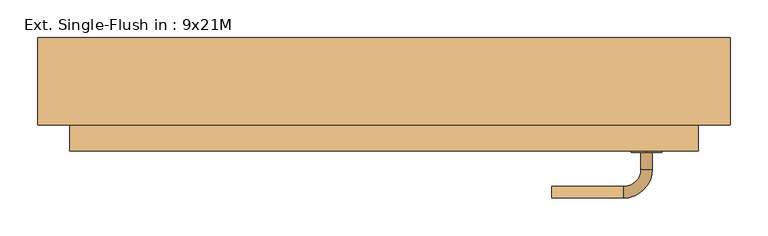
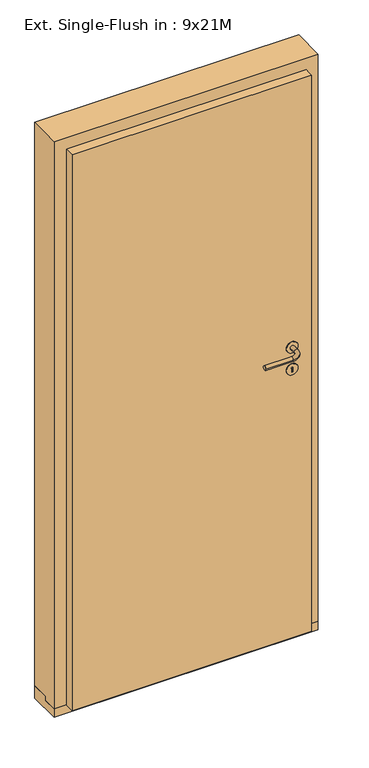
"""IFC4 building model written with IfcOpenShell, lengths in millimetres: door geometry, Ext. Single-Flush in : 9x21M."""

import ifcopenshell
import ifcopenshell.guid

model = None  # the IFC model being written
_history = None  # IfcOwnerHistory: only IFC2X3 demands one
_inside = {}  # id of a spatial element -> (the spatial element, [elements in it])
_under = {}  # id of a project, library or spatial element -> (it, [spatial elements below it])
_declared = {}  # id of a project -> (the project, [libraries it declares])
_typed = {}  # id of a type object -> (the type object, [elements of that type])
_made_of = {}  # id of a material, layer set ... -> (it, [elements and type objects made of it])


def new_model(schema):
    """Start an empty IFC model of exactly this schema.

    Asked for "IFC4X3", IfcOpenShell would pick the latest addendum, in which some entities
    have other attributes; the version numbers below select the first issue.
    IFC2X3 requires an IfcOwnerHistory on every rooted entity: one is made here for all.
    """
    global model, _history
    if schema == "IFC4X3":
        model = ifcopenshell.file(schema_version=(4, 3, 0, 0))
    else:
        model = ifcopenshell.file(schema=schema)
    _inside.clear()
    _under.clear()
    _declared.clear()
    _typed.clear()
    _made_of.clear()
    _history = None
    if model.schema == "IFC2X3":
        org = make("IfcOrganization", Name="unknown")
        user = make(
            "IfcPersonAndOrganization",
            ThePerson=make("IfcPerson", FamilyName="unknown"),
            TheOrganization=org,
        )
        app = make(
            "IfcApplication",
            ApplicationDeveloper=org,
            Version="unknown",
            ApplicationFullName="unknown",
            ApplicationIdentifier="unknown",
        )
        _history = make(
            "IfcOwnerHistory",
            OwningUser=user,
            OwningApplication=app,
            ChangeAction="ADDED",
            CreationDate=0,
        )
    return model


def make(cls, **values):
    """One entity of the class cls with the attributes given. An attribute that is None is left unset."""
    return model.create_entity(
        cls, **{name: value for name, value in values.items() if value is not None}
    )


def rooted(cls, **values):
    """An entity with a GlobalId (a new one), such as an element, a storey or a relation."""
    return make(cls, GlobalId=ifcopenshell.guid.new(), OwnerHistory=_history, **values)


def si_unit(unit_type, name, prefix=None):
    """IfcSIUnit, for example si_unit("LENGTHUNIT", "METRE", prefix="MILLI")."""
    return make("IfcSIUnit", UnitType=unit_type, Prefix=prefix, Name=name)


def assignment(units):
    """IfcUnitAssignment: the units of a project."""
    return None if units is None else make("IfcUnitAssignment", Units=units)


def point(xyz):
    """IfcCartesianPoint."""
    return None if xyz is None else make("IfcCartesianPoint", Coordinates=xyz)


def direction(xyz):
    """IfcDirection."""
    return None if xyz is None else make("IfcDirection", DirectionRatios=xyz)


def frame(location, z_axis=None, x_axis=None):
    """IfcAxis2Placement3D, a coordinate frame: its origin and axes. An axis left out is left unset."""
    return make(
        "IfcAxis2Placement3D",
        Location=point(location),
        Axis=direction(z_axis),
        RefDirection=direction(x_axis),
    )


def frame_2d(location, x_axis=None):
    """IfcAxis2Placement2D, a coordinate frame in the plane: its origin and x axis."""
    return make(
        "IfcAxis2Placement2D", Location=point(location), RefDirection=direction(x_axis)
    )


def origin():
    """The frame at (0, 0, 0) with its axes left unset."""
    return frame((0.0, 0.0, 0.0))


def place(relative_to, where):
    """IfcLocalPlacement: puts the frame where relative to a parent placement (None: the world)."""
    return make(
        "IfcLocalPlacement", PlacementRelTo=relative_to, RelativePlacement=where
    )


def context(
    kind, dimensions, precision=None, world=None, true_north=None, identifier=None
):
    """IfcGeometricRepresentationContext, for example the 3D "Model" context."""
    return make(
        "IfcGeometricRepresentationContext",
        ContextIdentifier=identifier,
        ContextType=kind,
        CoordinateSpaceDimension=dimensions,
        Precision=precision,
        WorldCoordinateSystem=world,
        TrueNorth=true_north,
    )


def project(units=None, contexts=None):
    """IfcProject with its units and contexts."""
    return rooted(
        "IfcProject",
        Name="project",
        RepresentationContexts=contexts,
        UnitsInContext=assignment(units),
    )


def spatial(cls, under=None, at=None, **own):
    """A site, building, storey or space (cls), placed at a placement, below another one or the project."""
    s = rooted(cls, ObjectPlacement=at, **own)
    if under is not None:
        _under.setdefault(under.id(), (under, []))[1].append(s)
    return s


def polyline(points):
    """IfcPolyline through the points."""
    return make("IfcPolyline", Points=[point(p) for p in points])


def circle_curve(where, radius):
    """IfcCircle in the frame where."""
    return make("IfcCircle", Position=where, Radius=radius)


def ellipse_curve(where, semi_axis1, semi_axis2):
    """IfcEllipse in the frame where."""
    return make(
        "IfcEllipse", Position=where, SemiAxis1=semi_axis1, SemiAxis2=semi_axis2
    )


def trimmed(basis, trim1, trim2, sense, master):
    """IfcTrimmedCurve: the piece of a basis curve between two trims."""
    return make(
        "IfcTrimmedCurve",
        BasisCurve=basis,
        Trim1=trim1,
        Trim2=trim2,
        SenseAgreement=sense,
        MasterRepresentation=master,
    )


def segment(curve, same_sense, transition):
    """IfcCompositeCurveSegment."""
    return make(
        "IfcCompositeCurveSegment",
        Transition=transition,
        SameSense=same_sense,
        ParentCurve=curve,
    )


def composite_curve(segments, self_intersect=None):
    """IfcCompositeCurve: segments joined end to end."""
    return make("IfcCompositeCurve", Segments=segments, SelfIntersect=self_intersect)


def outline(outer, holes=None, kind="AREA"):
    """IfcArbitraryClosedProfileDef: a profile drawn as a closed curve; with holes, ...WithVoids."""
    if holes is None:
        return make("IfcArbitraryClosedProfileDef", ProfileType=kind, OuterCurve=outer)
    return make(
        "IfcArbitraryProfileDefWithVoids",
        ProfileType=kind,
        OuterCurve=outer,
        InnerCurves=holes,
    )


def extrude(swept, where, along, depth):
    """IfcExtrudedAreaSolid: the profile swept, set in the frame where, extruded along a direction by depth."""
    return make(
        "IfcExtrudedAreaSolid",
        SweptArea=swept,
        Position=where,
        ExtrudedDirection=direction(along),
        Depth=depth,
    )


def faces_of(points, faces, orient=None, outer=None):
    """IfcFace entities. A face is a list of loops; a loop is a list of indices into points, from 0.

    orient and outer hold one flag for each loop. By default every Orientation is true, the
    first loop of a face is its IfcFaceOuterBound and the others are IfcFaceBound.
    """
    made = []
    for i, loops in enumerate(faces):
        bounds = []
        for j, loop in enumerate(loops):
            is_outer = j == 0 if outer is None else outer[i][j]
            bounds.append(
                make(
                    "IfcFaceOuterBound" if is_outer else "IfcFaceBound",
                    Bound=make("IfcPolyLoop", Polygon=[points[k] for k in loop]),
                    Orientation=True if orient is None else orient[i][j],
                )
            )
        made.append(make("IfcFace", Bounds=bounds))
    return made


def faceted_brep(points, faces, orient=None, outer=None, voids=None):
    """IfcFacetedBrep: a solid bounded by flat faces; with voids (closed shells), ...WithVoids."""
    shared = [point(p) for p in points]
    hull = make("IfcClosedShell", CfsFaces=faces_of(shared, faces, orient, outer))
    if voids is None:
        return make("IfcFacetedBrep", Outer=hull)
    return make(
        "IfcFacetedBrepWithVoids",
        Outer=hull,
        Voids=[
            make(cls, CfsFaces=faces_of(shared, fs, o, b)) for cls, fs, o, b in voids
        ],
    )


def shape(context_of_items, identifier, shape_type, items):
    """IfcShapeRepresentation: the items that make up one representation, for example the "Body"."""
    return make(
        "IfcShapeRepresentation",
        ContextOfItems=context_of_items,
        RepresentationIdentifier=identifier,
        RepresentationType=shape_type,
        Items=items,
    )


def source(mapping_origin, context_of_items, identifier, shape_type, items):
    """IfcRepresentationMap: a shape defined once, which mapped items show again and again."""
    return make(
        "IfcRepresentationMap",
        MappingOrigin=mapping_origin,
        MappedRepresentation=shape(context_of_items, identifier, shape_type, items),
    )


def transform(
    local_origin,
    x_axis=None,
    y_axis=None,
    z_axis=None,
    scale=None,
    scale2=None,
    scale3=None,
    uniform=True,
):
    """IfcCartesianTransformationOperator3D, or its non-uniform kind. x_axis, y_axis, z_axis: its Axis1, 2, 3."""
    if uniform:
        return make(
            "IfcCartesianTransformationOperator3D",
            Axis1=direction(x_axis),
            Axis2=direction(y_axis),
            LocalOrigin=point(local_origin),
            Scale=scale,
            Axis3=direction(z_axis),
        )
    return make(
        "IfcCartesianTransformationOperator3DnonUniform",
        Axis1=direction(x_axis),
        Axis2=direction(y_axis),
        LocalOrigin=point(local_origin),
        Scale=scale,
        Axis3=direction(z_axis),
        Scale2=scale2,
        Scale3=scale3,
    )


def mapped(mapping_source, mapping_target):
    """IfcMappedItem: shows the shape of a source again, moved by a transform."""
    return make(
        "IfcMappedItem", MappingSource=mapping_source, MappingTarget=mapping_target
    )


def made_of(thing, what):
    """Note that an element or type object is made of a material, layer set ...; save() writes the relation."""
    if what is not None:
        _made_of.setdefault(what.id(), (what, []))[1].append(thing)
    return thing


def element(
    cls,
    number,
    at=None,
    inside=None,
    cuts=None,
    type_object=None,
    material=None,
    context=None,
    identifier="Body",
    shape_type=None,
    held_by="IfcProductDefinitionShape",
    body=None,
    shapes=None,
    **own,
):
    """One element of the class cls, such as IfcWall. Its Tag is "e" and its number.

    at: its placement. inside: the storey or other place that contains it. cuts: it is an
    opening in that element (IfcRelVoidsElement). A single representation is given by context,
    identifier, shape_type and body (its items); several are given by shapes. held_by: the class
    of the entity that holds the representations. save() writes the other relations.
    """
    e = rooted(cls, Tag="e%d" % number, ObjectPlacement=at, **own)
    if body is not None:
        shapes = [shape(context, identifier, shape_type, body)]
    if shapes is not None:
        e.Representation = make(held_by, Representations=shapes)
    if inside is not None:
        _inside.setdefault(inside.id(), (inside, []))[1].append(e)
    if cuts is not None:
        rooted(
            "IfcRelVoidsElement", RelatingBuildingElement=cuts, RelatedOpeningElement=e
        )
    if type_object is not None:
        _typed.setdefault(type_object.id(), (type_object, []))[1].append(e)
    return made_of(e, material)


def aggregate(whole, parts):
    """IfcRelAggregates: a whole, such as a stair, and the parts it consists of."""
    return rooted("IfcRelAggregates", RelatingObject=whole, RelatedObjects=parts)


def save(model, path):
    """Write the relations noted so far, then the file.

    IfcRelAggregates (storeys below a building ...), IfcRelContainedInSpatialStructure (elements
    in a storey), IfcRelDefinesByType, IfcRelAssociatesMaterial and IfcRelDeclares: one each for
    every whole, place, type object, material and project.
    """
    for whole, parts in _under.values():
        aggregate(whole, parts)
    for where, things in _inside.values():
        rooted(
            "IfcRelContainedInSpatialStructure",
            RelatedElements=things,
            RelatingStructure=where,
        )
    for kind, things in _typed.values():
        rooted("IfcRelDefinesByType", RelatedObjects=things, RelatingType=kind)
    for what, things in _made_of.values():
        rooted("IfcRelAssociatesMaterial", RelatedObjects=things, RelatingMaterial=what)
    for by, libraries in _declared.values():
        rooted("IfcRelDeclares", RelatingContext=by, RelatedDefinitions=libraries)
    model.write(path)


def plane_surface(at):
    """IfcPlane: the flat surface through the origin of the frame at, square to its z axis."""
    return make("IfcPlane", Position=at)


def cylinder_surface(at, radius):
    """IfcCylindricalSurface: all points at the distance radius from the z axis of the frame at."""
    return make("IfcCylindricalSurface", Position=at, Radius=radius)


def revolved_surface(curve, axis_point, axis_direction):
    """IfcSurfaceOfRevolution: the curve turned about the line through axis_point along axis_direction."""
    return make(
        "IfcSurfaceOfRevolution",
        SweptCurve=make("IfcArbitraryOpenProfileDef", ProfileType="CURVE", Curve=curve),
        AxisPosition=make("IfcAxis1Placement", Location=point(axis_point), Axis=direction(axis_direction)),
    )


def advanced_brep(points, edges, surfaces, faces):
    """IfcAdvancedBrep: a solid bounded by faces that lie on surfaces and meet in shared edges.

    An edge is (start, end): straight between two places in points (the first is 0);
    or (start, end, curve); or (start, end, curve, False) where it runs against its curve.
    A face is (place in surfaces, loops), or (place, loops, False) where it looks against
    its surface's normal. A loop lists edges by number (the first is 1), with a minus sign
    where the edge is run from its end to its start. The first loop is the outer one.
    """
    corners = [point(p) for p in points]
    vertices = [make("IfcVertexPoint", VertexGeometry=c) for c in corners]
    made = []
    for start, end, *more in edges:
        made.append(
            make(
                "IfcEdgeCurve",
                EdgeStart=vertices[start],
                EdgeEnd=vertices[end],
                EdgeGeometry=more[0] if more else make("IfcPolyline", Points=[corners[start], corners[end]]),
                SameSense=more[1] if len(more) > 1 else True,
            )
        )
    hull = []
    for where, loops, *sense in faces:
        bounds = []
        for j, loop in enumerate(loops):
            ring = [make("IfcOrientedEdge", EdgeElement=made[abs(k) - 1], Orientation=k > 0) for k in loop]
            bounds.append(
                make(
                    "IfcFaceOuterBound" if j == 0 else "IfcFaceBound",
                    Bound=make("IfcEdgeLoop", EdgeList=ring),
                    Orientation=True,
                )
            )
        hull.append(make("IfcAdvancedFace", Bounds=bounds, FaceSurface=surfaces[where], SameSense=sense[0] if sense else True))
    return make("IfcAdvancedBrep", Outer=make("IfcClosedShell", CfsFaces=hull))


def ext_single_flush_in_9x21m_d6ab10a1(model_context):
    return source(origin(), model_context, "Body", "SolidModel", [
        extrude(outline(composite_curve([segment(trimmed(circle_curve(frame_2d((1090.0, 346.0)), 20.0), [point((1070.0, 346.0))], [point((1110.0, 346.0))], False, "CARTESIAN"), True, "CONTINUOUS"), segment(trimmed(circle_curve(frame_2d((1090.0, 346.0)), 20.0), [point((1110.0, 346.0))], [point((1070.0, 346.0))], False, "CARTESIAN"), True, "CONTINUOUS")], self_intersect=False)), frame((0.0, 33.0, 0.0), z_axis=(0.0, 1.0, 0.0), x_axis=(0.0, 0.0, 1.0)), (0.0, 0.0, 1.0), 2.0),
        advanced_brep(
        [(353.5, 33.0, 1090.0), (338.5, 33.0, 1090.0), (353.5, 10.5, 1090.0), (338.5, 10.5, 1090.0), (316.0, -12.0, 1090.0), (316.0, -27.0, 1090.0), (221.0, -27.0, 1090.0), (221.0, -12.0, 1090.0)],
        [
            (0, 1, circle_curve(frame((346.0, 33.0, 1090.0), z_axis=(0.0, 1.0, 0.0), x_axis=(-1.0, 0.0, 0.0)), 7.5)),
            (1, 0, circle_curve(frame((346.0, 33.0, 1090.0), z_axis=(0.0, 1.0, 0.0), x_axis=(-1.0, 0.0, 0.0)), 7.5)),
            (0, 2),
            (2, 3, circle_curve(frame((346.0, 10.5, 1090.0), z_axis=(0.0, 1.0, 0.0), x_axis=(-1.0, 0.0, 0.0)), 7.5)),
            (3, 1),
            (3, 2, circle_curve(frame((346.0, 10.5, 1090.0), z_axis=(0.0, 1.0, 0.0), x_axis=(-1.0, 0.0, 0.0)), 7.5)),
            (4, 3, circle_curve(frame((316.0, 10.5, 1090.0), z_axis=(0.0, 0.0, 1.0), x_axis=(1.0, 0.0, 0.0)), 22.5)),
            (2, 5, circle_curve(frame((316.0, 10.5, 1090.0), z_axis=(0.0, 0.0, -1.0), x_axis=(1.0, 0.0, 0.0)), 37.5)),
            (5, 4, circle_curve(frame((316.0, -19.5, 1090.0), z_axis=(1.0, 0.0, 0.0), x_axis=(0.0, 1.0, 0.0)), 7.5)),
            (4, 5, circle_curve(frame((316.0, -19.5, 1090.0), z_axis=(1.0, 0.0, 0.0), x_axis=(0.0, 1.0, 0.0)), 7.5)),
            (5, 6),
            (6, 7, circle_curve(frame((221.0, -19.5, 1090.0), z_axis=(1.0, 0.0, 0.0), x_axis=(0.0, 1.0, 0.0)), 7.5)),
            (7, 4),
            (7, 6, circle_curve(frame((221.0, -19.5, 1090.0), z_axis=(1.0, 0.0, 0.0), x_axis=(0.0, 1.0, 0.0)), 7.5)),
        ],
        [
            plane_surface(frame((346.0, 33.0, 1090.0), z_axis=(0.0, 1.0, 0.0), x_axis=(0.0, 0.0, -1.0))),
            cylinder_surface(frame((346.0, 33.0, 1090.0), z_axis=(0.0, 1.0, 0.0), x_axis=(-1.0, 0.0, 0.0)), 7.5),
            revolved_surface(trimmed(ellipse_curve(frame((346.0, 10.5, 1090.0), z_axis=(0.0, 1.0, 0.0), x_axis=(-1.0, 0.0, 0.0)), 7.5, 7.5), [point((353.5, 10.5, 1090.0))], [point((338.5, 10.5, 1090.0))], True, "CARTESIAN"), (316.0, 10.5, 1090.0), (0.0, 0.0, -1.0)),
            revolved_surface(trimmed(ellipse_curve(frame((346.0, 10.5, 1090.0), z_axis=(0.0, 1.0, 0.0), x_axis=(-1.0, 0.0, 0.0)), 7.5, 7.5), [point((338.5, 10.5, 1090.0))], [point((353.5, 10.5, 1090.0))], True, "CARTESIAN"), (316.0, 10.5, 1090.0), (0.0, 0.0, -1.0)),
            cylinder_surface(frame((316.0, -19.5, 1090.0), z_axis=(1.0, 0.0, 0.0), x_axis=(0.0, 1.0, 0.0)), 7.5),
            plane_surface(frame((221.0, -19.5, 1090.0), z_axis=(-1.0, 0.0, 0.0), x_axis=(0.0, 0.0, -1.0))),
        ],
        [
            (0, [[1, 2]]),
            (1, [[-1, 3, 4, 5]]),
            (1, [[-2, -5, 6, -3]]),
            (2, [[7, -4, 8, 9]]),
            (3, [[-8, -6, -7, 10]]),
            (4, [[-9, 11, 12, 13]]),
            (4, [[-10, -13, 14, -11]]),
            (5, [[-14, -12]]),
        ],
    ),
        extrude(outline(composite_curve([segment(trimmed(circle_curve(frame_2d((1010.0, 346.0)), 20.0), [point((990.0, 346.0))], [point((1030.0, 346.0))], False, "CARTESIAN"), True, "CONTINUOUS"), segment(trimmed(circle_curve(frame_2d((1010.0, 346.0)), 20.0), [point((1030.0, 346.0))], [point((990.0, 346.0))], False, "CARTESIAN"), True, "CONTINUOUS")], self_intersect=False), holes=[composite_curve([segment(polyline([(1012.4019238, 347.5), (1000.0, 347.5), (1000.0, 344.5), (1012.4019238, 344.5)]), True, "CONTINUOUS"), segment(trimmed(circle_curve(frame_2d((1015.0, 346.0)), 3.0), [point((1012.4019238, 344.5))], [point((1012.4019238, 347.5))], True, "CARTESIAN"), True, "CONTINUOUS")], self_intersect=False)]), frame((0.0, 33.0, 0.0), z_axis=(0.0, 1.0, 0.0), x_axis=(0.0, 0.0, 1.0)), (0.0, 0.0, 1.0), 2.0),
        extrude(outline(composite_curve([segment(trimmed(circle_curve(frame_2d((1090.0, 346.0)), 20.0), [point((1070.0, 346.0))], [point((1110.0, 346.0))], False, "CARTESIAN"), True, "CONTINUOUS"), segment(trimmed(circle_curve(frame_2d((1090.0, 346.0)), 20.0), [point((1110.0, 346.0))], [point((1070.0, 346.0))], False, "CARTESIAN"), True, "CONTINUOUS")], self_intersect=False)), frame((0.0, 85.0, 0.0), z_axis=(0.0, 1.0, 0.0), x_axis=(0.0, 0.0, 1.0)), (0.0, 0.0, 1.0), 2.0),
        advanced_brep(
        [(353.5, 87.0, 1090.0), (338.5, 87.0, 1090.0), (338.5, 109.5, 1090.0), (353.5, 109.5, 1090.0), (316.0, 132.0, 1090.0), (316.0, 147.0, 1090.0), (221.0, 132.0, 1090.0), (221.0, 147.0, 1090.0)],
        [
            (0, 1, circle_curve(frame((346.0, 87.0, 1090.0), z_axis=(0.0, -1.0, 0.0), x_axis=(-1.0, 0.0, 0.0)), 7.5)),
            (1, 0, circle_curve(frame((346.0, 87.0, 1090.0), z_axis=(0.0, -1.0, 0.0), x_axis=(-1.0, 0.0, 0.0)), 7.5)),
            (1, 2),
            (2, 3, circle_curve(frame((346.0, 109.5, 1090.0), z_axis=(0.0, -1.0, 0.0), x_axis=(-1.0, 0.0, 0.0)), 7.5)),
            (3, 0),
            (3, 2, circle_curve(frame((346.0, 109.5, 1090.0), z_axis=(0.0, -1.0, 0.0), x_axis=(-1.0, 0.0, 0.0)), 7.5)),
            (4, 5, circle_curve(frame((316.0, 139.5, 1090.0), z_axis=(1.0, 0.0, 0.0), x_axis=(0.0, -1.0, 0.0)), 7.5)),
            (5, 3, circle_curve(frame((316.0, 109.5, 1090.0), z_axis=(0.0, 0.0, -1.0), x_axis=(1.0, 0.0, 0.0)), 37.5)),
            (2, 4, circle_curve(frame((316.0, 109.5, 1090.0), z_axis=(0.0, 0.0, 1.0), x_axis=(1.0, 0.0, 0.0)), 22.5)),
            (5, 4, circle_curve(frame((316.0, 139.5, 1090.0), z_axis=(1.0, 0.0, 0.0), x_axis=(0.0, -1.0, 0.0)), 7.5)),
            (4, 6),
            (6, 7, circle_curve(frame((221.0, 139.5, 1090.0), z_axis=(1.0, 0.0, 0.0), x_axis=(0.0, -1.0, 0.0)), 7.5)),
            (7, 5),
            (7, 6, circle_curve(frame((221.0, 139.5, 1090.0), z_axis=(1.0, 0.0, 0.0), x_axis=(0.0, -1.0, 0.0)), 7.5)),
        ],
        [
            plane_surface(frame((346.0, 87.0, 1090.0), z_axis=(0.0, -1.0, 0.0), x_axis=(0.0, 0.0, -1.0))),
            cylinder_surface(frame((346.0, 87.0, 1090.0), z_axis=(0.0, -1.0, 0.0), x_axis=(-1.0, 0.0, 0.0)), 7.5),
            revolved_surface(trimmed(ellipse_curve(frame((346.0, 109.5, 1090.0), z_axis=(0.0, 1.0, 0.0), x_axis=(-1.0, 0.0, 0.0)), 7.5, 7.5), [point((353.5, 109.5, 1090.0))], [point((338.5, 109.5, 1090.0))], True, "CARTESIAN"), (316.0, 109.5, 1090.0), (0.0, 0.0, -1.0)),
            revolved_surface(trimmed(ellipse_curve(frame((346.0, 109.5, 1090.0), z_axis=(0.0, 1.0, 0.0), x_axis=(-1.0, 0.0, 0.0)), 7.5, 7.5), [point((338.5, 109.5, 1090.0))], [point((353.5, 109.5, 1090.0))], True, "CARTESIAN"), (316.0, 109.5, 1090.0), (0.0, 0.0, -1.0)),
            cylinder_surface(frame((316.0, 139.5, 1090.0), z_axis=(1.0, 0.0, 0.0), x_axis=(0.0, -1.0, 0.0)), 7.5),
            plane_surface(frame((221.0, 139.5, 1090.0), z_axis=(-1.0, 0.0, 0.0), x_axis=(0.0, 0.0, -1.0))),
        ],
        [
            (0, [[1, 2]]),
            (1, [[3, 4, 5, -2]]),
            (1, [[-5, 6, -3, -1]]),
            (2, [[7, 8, -4, 9]]),
            (3, [[10, -9, -6, -8]]),
            (4, [[11, 12, 13, -7]]),
            (4, [[-13, 14, -11, -10]]),
            (5, [[-12, -14]]),
        ],
    ),
        extrude(outline(composite_curve([segment(trimmed(circle_curve(frame_2d((1010.0, 346.0)), 20.0), [point((990.0, 346.0))], [point((1030.0, 346.0))], False, "CARTESIAN"), True, "CONTINUOUS"), segment(trimmed(circle_curve(frame_2d((1010.0, 346.0)), 20.0), [point((1030.0, 346.0))], [point((990.0, 346.0))], False, "CARTESIAN"), True, "CONTINUOUS")], self_intersect=False), holes=[composite_curve([segment(polyline([(1012.4019238, 347.5), (1000.0, 347.5), (1000.0, 344.5), (1012.4019238, 344.5)]), True, "CONTINUOUS"), segment(trimmed(circle_curve(frame_2d((1015.0, 346.0)), 3.0), [point((1012.4019238, 344.5))], [point((1012.4019238, 347.5))], True, "CARTESIAN"), True, "CONTINUOUS")], self_intersect=False)]), frame((0.0, 85.0, 0.0), z_axis=(0.0, 1.0, 0.0), x_axis=(0.0, 0.0, 1.0)), (0.0, 0.0, 1.0), 2.0),
        faceted_brep([(-414.0, 69.0, 2058.0), (414.0, 69.0, 2058.0), (414.0, 69.0, 30.0), (456.0, 69.0, 30.0), (456.0, 69.0, 2100.0), (-456.0, 69.0, 2100.0), (-456.0, 69.0, 30.0), (-414.0, 69.0, 30.0), (414.0, 119.0, 2058.0), (414.0, 119.0, 45.0), (414.0, 119.0, 30.0), (-456.0, 119.0, 30.0), (-414.0, 119.0, 30.0), (456.0, 119.0, 30.0), (456.0, 184.0, 2100.0), (456.0, 119.0, 45.0), (456.0, 184.0, 45.0), (-456.0, 184.0, 2100.0), (-456.0, 184.0, 45.0), (-456.0, 119.0, 45.0), (-414.0, 119.0, 2058.0), (-414.0, 119.0, 45.0), (399.0, 184.0, 45.0), (399.0, 184.0, 2043.0), (-399.0, 184.0, 2043.0), (-399.0, 184.0, 45.0), (-399.0, 119.0, 45.0), (399.0, 119.0, 45.0), (399.0, 119.0, 2043.0), (-399.0, 119.0, 2043.0)], [[[0, 1, 2, 3, 4, 5, 6, 7]], [[1, 8, 9, 10, 2]], [[11, 12, 7, 6]], [[10, 13, 3, 2]], [[14, 4, 3, 13, 15, 16]], [[5, 17, 18, 19, 11, 6]], [[20, 0, 7, 12, 21]], [[17, 14, 16, 22, 23, 24, 25, 18]], [[21, 19, 18, 25, 26]], [[15, 9, 27, 22, 16]], [[12, 11, 19, 21]], [[13, 10, 9, 15]], [[28, 23, 22, 27]], [[24, 29, 26, 25]], [[29, 28, 27, 9, 8, 20, 21, 26]], [[5, 4, 14, 17]], [[24, 23, 28, 29]], [[1, 0, 20, 8]]]),
        extrude(outline(polyline([(-414.0, 85.0), (414.0, 85.0), (414.0, 35.0), (-414.0, 35.0), (-414.0, 85.0)])), frame((0.0, 0.0, 30.0), z_axis=(0.0, 0.0, 1.0), x_axis=(1.0, 0.0, 0.0)), (0.0, 0.0, 1.0), 2028.0),
        extrude(outline(polyline([(69.0, 30.0), (119.0, 30.0), (119.0, 45.0), (184.0, 45.0), (184.0, 0.0), (69.0, 0.0), (69.0, 30.0)])), frame((-456.0, 0.0, 0.0), z_axis=(1.0, 0.0, 0.0), x_axis=(0.0, 1.0, 0.0)), (0.0, 0.0, 1.0), 912.0),
    ])


if __name__ == "__main__":
    model = new_model("IFC4")
    model_context = context("Model", 3, world=origin())
    ifc_project = project(units=[si_unit("LENGTHUNIT", "METRE", prefix="MILLI")], contexts=[model_context])
    site = spatial("IfcSite", under=ifc_project)
    building = spatial("IfcBuilding", under=site)
    placement = place(None, origin())
    ext_single_flush_in_9x21m_shape = ext_single_flush_in_9x21m_d6ab10a1(model_context)
    element("IfcDoor", 1, ObjectType="Ext. Single-Flush in : 9x21M", at=placement, inside=building, context=model_context, shape_type="MappedRepresentation", body=[
        mapped(ext_single_flush_in_9x21m_shape, transform((0.0, 0.0, 0.0), x_axis=(1.0, 0.0, 0.0), y_axis=(0.0, 1.0, 0.0), z_axis=(0.0, 0.0, 1.0))),
    ])
    save(model, "model.ifc")

# Revit data of these elements
# Type "Ext. Single-Flush in : 9x21M"
#   Type Mark = "62"
#   Sound Rating = ""
#   Opening Side [instance default] = "in"
#   Hinge Side [instance default] = ""
#   Creator Build [instance default] = "2017.0301.0"
#   Creator Organization [instance default] = "© Danish Educational Content"
#   Creator Name [instance default] = "© Erik Falck Jørgensen"
#   Analytic Construction = "<None>"
#   length#5 = 912 mm
#   length#4 = 120 mm
#   length#3 = 30 mm
#   length#2 = 57 mm
#   length#1 = 0 mm
#   Thickness = 50 mm
#   Seal Width = 12 mm
#   Rough Width = 912 mm
#   Rough Height = 2100 mm
#   Rebate Depth = 50 mm
#   Rabbet Width = 15 mm
#   Rabbet Depth = 50 mm
#   Height = 2088 mm
#   Width = 888 mm
#   Handle From Side = 110 mm
#   Handle From Bottom = 1090 mm
#   Exterior Direction [instance default] = 0.00°
#   Case Depth = 115 mm
#   Case Width = 45 mm
#   Threshold = yes
#   Sealing = no
#   Hinging = yes
#   Wall Closure = 1
#   Function = 1
#   Panel = none
#   Handle Finish = none
#   Handle = element 628255
#   Case/Transom = none
#   Assembly Code = ""
# Element 1 (IfcDoor, "Ext. Single-Flush in : 9x21M")
#   Materials on its faces: "Stainless Steel, Polished", "Default Frame/Mullion (Interior/Exterior)", "Default Door Panel (Exterior/Interior)"
# Materials
#   "Stainless Steel, Polished": class "Metal", colour RGB 180 180 180, transparency 0, Description = "Rustfri stål, poleret", Cost = 0
#   "Default Frame/Mullion (Interior/Exterior)": class "Generic", colour RGB 205 205 205, transparency 0, Description = "Udefineret karm/ramme materiale", Cost = 0
#   "Default Door Panel (Exterior/Interior)": class "Generic", colour RGB 205 205 205, transparency 0, Description = "Udefineret dørplade materiale", Cost = 0
